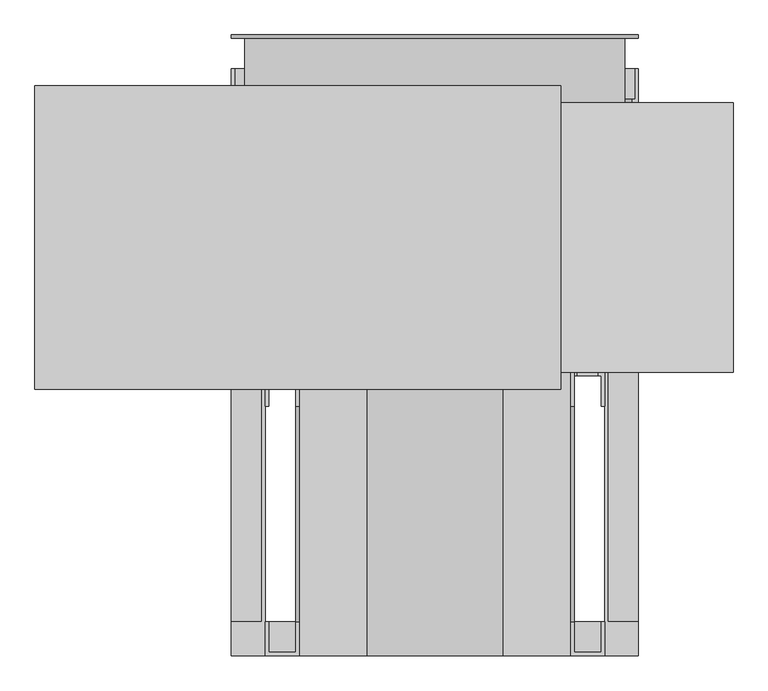
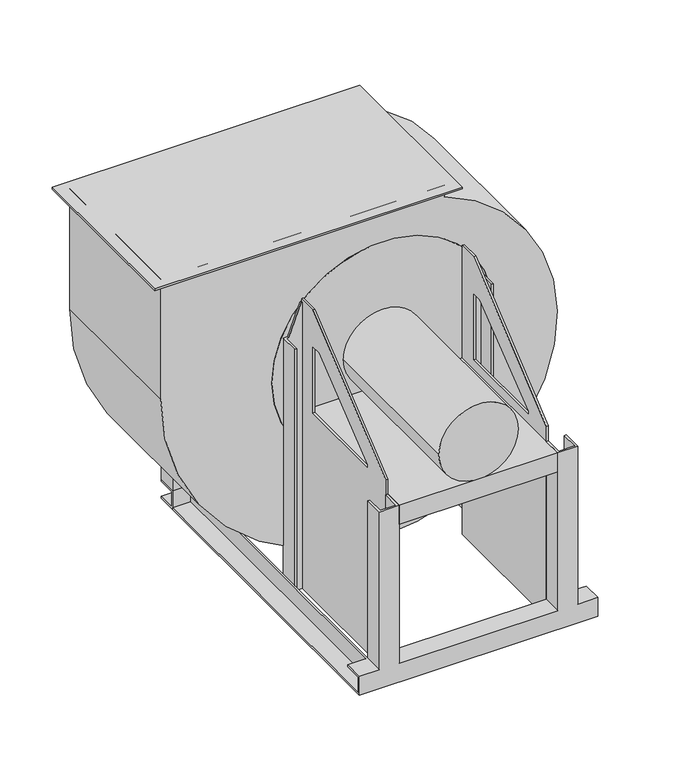
"""IFC4 building model written with IfcOpenShell, lengths in millimetres: proxy geometry, ВЕЗА_Вентилятор ВРАН : ВРАН6-056."""

from ifc_helpers import new_model, si_unit, point, frame, frame_2d, origin, place, context, project, spatial, polyline, circle_curve, trimmed, segment, composite_curve, outline, extrude, faceted_brep, source, transform, mapped, element, save


def mechanical_equipment_cec6a2f8(model_context):
    return source(origin(), model_context, "Body", "SolidModel", [
        extrude(outline(polyline([(185.5, -223.5), (-589.5, -223.5), (-589.5, 223.5), (185.5, 223.5), (185.5, -223.5)])), frame((0.0, 0.0, 940.0), z_axis=(0.0, 0.0, 1.0), x_axis=(1.0, 0.0, 0.0)), (0.0, 0.0, 1.0), 5.0),
        extrude(outline(composite_curve([segment(trimmed(circle_curve(frame_2d((625.0, 0.5002234)), 560.0002234), [point((625.0, -559.5))], [point((65.0, 0.0))], False, "CARTESIAN"), True, "CONTINUOUS"), segment(trimmed(circle_curve(frame_2d((504.1653304, 0.3189338)), 439.1654462), [point((65.0, 0.0))], [point((915.0, 155.5))], False, "CARTESIAN"), True, "CONTINUOUS"), segment(polyline([(915.0, 155.5), (945.0, 155.5), (945.0, -559.5), (625.0, -559.5)]), True, "CONTINUOUS")], self_intersect=False), holes=[composite_curve([segment(trimmed(circle_curve(frame_2d((570.0, 0.0)), 280.0), [point((570.0, -280.0))], [point((570.0, 280.0))], True, "CARTESIAN"), True, "CONTINUOUS"), segment(trimmed(circle_curve(frame_2d((570.0, 0.0)), 280.0), [point((570.0, 280.0))], [point((570.0, -280.0))], True, "CARTESIAN"), True, "CONTINUOUS")], self_intersect=False)]), frame((0.0, -198.5, 0.0), z_axis=(0.0, 1.0, 0.0), x_axis=(0.0, 0.0, 1.0)), (0.0, 0.0, 1.0), 397.0),
        faceted_brep([(-300.0, -611.5, 5.0), (-300.0, 198.5, 5.0), (-300.0, 198.5, 0.0), (-300.0, -616.5, 0.0), (-300.0, -616.5, 50.0), (-300.0, -566.5, 50.0), (-300.0, -566.5, 45.0), (-300.0, -611.5, 45.0), (300.0, -616.5, 50.0), (300.0, -616.5, 0.0), (300.0, 198.5, 0.0), (300.0, 198.5, 5.0), (300.0, -611.5, 5.0), (300.0, -611.5, 45.0), (300.0, -566.5, 45.0), (300.0, -566.5, 50.0), (-250.0, 198.5, 0.0), (-250.0, -566.5, 0.0), (250.0, -566.5, 0.0), (250.0, 198.5, 0.0), (-255.0, -566.5, 50.0), (-255.0, -566.5, 45.0), (255.0, -566.5, 45.0), (255.0, -566.5, 50.0), (-200.0, -566.5, 470.0), (-200.0, -566.5, 50.0), (200.0, -566.5, 50.0), (200.0, -566.5, 470.0), (205.0, -566.5, 470.0), (205.0, -566.5, 50.0), (245.0, -566.5, 50.0), (245.0, -566.5, 470.0), (250.0, -566.5, 470.0), (250.0, -566.5, 50.0), (-250.0, -566.5, 50.0), (-250.0, -566.5, 470.0), (-245.0, -566.5, 470.0), (-245.0, -566.5, 50.0), (-205.0, -566.5, 50.0), (-205.0, -566.5, 470.0), (205.0, -566.5, 5.0), (245.0, -566.5, 5.0), (245.0, -566.5, 45.0), (205.0, -566.5, 45.0), (-245.0, -566.5, 5.0), (-205.0, -566.5, 5.0), (-205.0, -566.5, 45.0), (-245.0, -566.5, 45.0), (-200.0, -566.5, 5.0), (200.0, -566.5, 5.0), (200.0, -566.5, 45.0), (-200.0, -566.5, 45.0), (-255.0, -611.5, 5.0), (-255.0, 198.5, 5.0), (255.0, 198.5, 5.0), (255.0, -611.5, 5.0), (205.0, -611.5, 5.0), (245.0, -611.5, 5.0), (-245.0, -611.5, 5.0), (-205.0, -611.5, 5.0), (-200.0, -611.5, 5.0), (200.0, -611.5, 5.0), (255.0, -611.5, 45.0), (-255.0, -611.5, 45.0), (205.0, -611.5, 45.0), (245.0, -611.5, 45.0), (-245.0, -611.5, 45.0), (-205.0, -611.5, 45.0), (-200.0, -611.5, 45.0), (200.0, -611.5, 45.0), (255.0, 198.5, 50.0), (250.0, 198.5, 50.0), (250.0, -616.5, 50.0), (-250.0, -616.5, 50.0), (-250.0, 198.5, 50.0), (-255.0, 198.5, 50.0), (205.0, -611.5, 50.0), (245.0, -611.5, 50.0), (-245.0, -611.5, 50.0), (-205.0, -611.5, 50.0), (-200.0, -616.5, 50.0), (200.0, -616.5, 50.0), (250.0, -616.5, 470.0), (200.0, -616.5, 470.0), (-200.0, -616.5, 470.0), (-250.0, -616.5, 470.0), (245.0, -611.5, 470.0), (205.0, -611.5, 470.0), (-205.0, -611.5, 470.0), (-245.0, -611.5, 470.0)], [[[0, 1, 2, 3, 4, 5, 6, 7]], [[8, 9, 10, 11, 12, 13, 14, 15]], [[10, 9, 3, 2, 16, 17, 18, 19]], [[5, 20, 21, 6]], [[14, 22, 23, 15]], [[24, 25, 26, 27, 28, 29, 30, 31, 32, 33, 18, 17, 34, 35, 36, 37, 38, 39], [40, 41, 42, 43], [44, 45, 46, 47], [48, 49, 50, 51]], [[1, 0, 52, 53]], [[54, 55, 12, 11]], [[40, 56, 57, 41]], [[44, 58, 59, 45]], [[48, 60, 61, 49]], [[12, 55, 62, 13]], [[7, 63, 52, 0]], [[56, 64, 65, 57]], [[58, 66, 67, 59]], [[60, 68, 69, 61]], [[6, 21, 63, 7]], [[13, 62, 22, 14]], [[64, 43, 42, 65]], [[66, 47, 46, 67]], [[68, 51, 50, 69]], [[15, 23, 70, 71, 33, 72, 8]], [[4, 73, 34, 74, 75, 20, 5]], [[29, 76, 77, 30]], [[37, 78, 79, 38]], [[25, 80, 81, 26]], [[8, 72, 82, 83, 81, 80, 84, 85, 73, 4, 3, 9]], [[70, 54, 11, 10, 19, 71]], [[70, 23, 22, 62, 55, 54]], [[19, 18, 33, 71]], [[75, 74, 16, 2, 1, 53]], [[53, 52, 63, 21, 20, 75]], [[74, 34, 17, 16]], [[83, 82, 32, 31, 86, 87, 28, 27]], [[84, 24, 39, 88, 89, 36, 35, 85]], [[86, 77, 76, 87]], [[31, 30, 77, 86]], [[41, 57, 65, 42]], [[82, 72, 33, 32]], [[27, 26, 81, 83]], [[49, 61, 69, 50]], [[43, 64, 56, 40]], [[87, 76, 29, 28]], [[35, 34, 73, 85]], [[47, 66, 58, 44]], [[89, 78, 37, 36]], [[88, 79, 78, 89]], [[39, 38, 79, 88]], [[45, 59, 67, 46]], [[51, 68, 60, 48]], [[84, 80, 25, 24]]]),
        extrude(outline(polyline([(-566.5, 0.0), (-566.5, 510.0420316), (-248.5420316, 770.0), (-198.5, 770.0), (-198.5, 0.0), (-566.5, 0.0)]), holes=[polyline([(-248.5, 495.0), (-248.5, 670.0), (-273.4504813, 670.0), (-486.5, 501.5949723), (-486.5, 495.0), (-248.5, 495.0)])]), frame((-205.0, 0.0, 0.0), z_axis=(1.0, 0.0, 0.0), x_axis=(0.0, 1.0, 0.0)), (0.0, 0.0, 1.0), 5.0),
        faceted_brep([(250.0, 198.5, 50.0), (250.0, 203.5, 50.0), (295.0, 203.5, 50.0), (295.0, 248.5, 50.0), (300.0, 248.5, 50.0), (300.0, 198.5, 50.0), (300.0, 198.5, 465.0), (289.966699, 198.5, 465.0), (258.2904546, 198.5, 370.0), (250.0, 198.5, 370.0), (300.0, 248.5, 465.0), (295.0, 248.5, 465.0), (295.0, 203.5, 465.0), (250.0, 203.5, 370.0), (258.2904546, 203.5, 370.0), (289.966699, 203.5, 465.0)], [[[0, 1, 2, 3, 4, 5]], [[5, 6, 7, 8, 9, 0]], [[4, 10, 6, 5]], [[3, 11, 10, 4]], [[2, 12, 11, 3]], [[1, 13, 14, 15, 12, 2]], [[0, 9, 13, 1]], [[14, 13, 9, 8]], [[8, 7, 15, 14]], [[7, 6, 10, 11, 12, 15]]]),
        faceted_brep([(-250.0, 198.5, 50.0), (-300.0, 198.5, 50.0), (-300.0, 248.5, 50.0), (-295.0, 248.5, 50.0), (-295.0, 203.5, 50.0), (-250.0, 203.5, 50.0), (-250.0, 203.5, 370.0), (-250.0, 198.5, 370.0), (-295.0, 203.5, 465.0), (-289.966699, 203.5, 465.0), (-258.2904546, 203.5, 370.0), (-295.0, 248.5, 465.0), (-300.0, 248.5, 465.0), (-300.0, 198.5, 465.0), (-258.2904546, 198.5, 370.0), (-289.966699, 198.5, 465.0)], [[[0, 1, 2, 3, 4, 5]], [[5, 6, 7, 0]], [[4, 8, 9, 10, 6, 5]], [[3, 11, 8, 4]], [[2, 12, 11, 3]], [[1, 13, 12, 2]], [[0, 7, 14, 15, 13, 1]], [[9, 8, 11, 12, 13, 15]], [[15, 14, 10, 9]], [[14, 7, 6, 10]]]),
        extrude(outline(polyline([(-566.5, 0.0), (-566.5, 510.0420316), (-248.5420316, 770.0), (-198.5, 770.0), (-198.5, 0.0), (-566.5, 0.0)]), holes=[polyline([(-248.5, 495.0), (-248.5, 670.0), (-273.4504813, 670.0), (-486.5, 501.5949723), (-486.5, 495.0), (-248.5, 495.0)])]), frame((200.0, 0.0, 0.0), z_axis=(1.0, 0.0, 0.0), x_axis=(0.0, 1.0, 0.0)), (0.0, 0.0, 1.0), 5.0),
        faceted_brep([(200.0, -198.5, 0.0), (250.0, -198.5, 0.0), (250.0, -248.5, 0.0), (245.0, -248.5, 0.0), (245.0, -203.5, 0.0), (200.0, -203.5, 0.0), (200.0, -198.5, 763.6095143), (208.75409, -198.5, 763.6095143), (240.0, -198.5, 680.0), (250.0, -198.5, 680.0), (250.0, -248.5, 680.0), (245.0, -248.5, 680.0), (245.0, -203.5, 680.0), (240.0, -203.5, 680.0), (208.75409, -203.5, 763.6095143), (200.0, -203.5, 763.6095143)], [[[0, 1, 2, 3, 4, 5]], [[0, 6, 7, 8, 9, 1]], [[1, 9, 10, 2]], [[2, 10, 11, 3]], [[3, 11, 12, 4]], [[4, 12, 13, 14, 15, 5]], [[5, 15, 6, 0]], [[7, 6, 15, 14]], [[14, 13, 8, 7]], [[13, 12, 11, 10, 9, 8]]]),
        faceted_brep([(-200.0, -198.5, 0.0), (-200.0, -203.5, 0.0), (-245.0, -203.5, 0.0), (-245.0, -248.5, 0.0), (-250.0, -248.5, 0.0), (-250.0, -198.5, 0.0), (-200.0, -198.5, 763.6095143), (-200.0, -203.5, 763.6095143), (-208.75409, -203.5, 763.6095143), (-240.0, -203.5, 680.0), (-245.0, -203.5, 680.0), (-245.0, -248.5, 680.0), (-250.0, -248.5, 680.0), (-250.0, -198.5, 680.0), (-240.0, -198.5, 680.0), (-208.75409, -198.5, 763.6095143)], [[[0, 1, 2, 3, 4, 5]], [[0, 6, 7, 1]], [[1, 7, 8, 9, 10, 2]], [[2, 10, 11, 3]], [[3, 11, 12, 4]], [[4, 12, 13, 5]], [[5, 13, 14, 15, 6, 0]], [[14, 13, 12, 11, 10, 9]], [[9, 8, 15, 14]], [[8, 7, 6, 15]]]),
        extrude(outline(polyline([(198.5, 50.0), (248.5, 50.0), (248.5, 45.0), (203.5, 45.0), (203.5, 5.0), (248.5, 5.0), (248.5, 0.0), (198.5, 0.0), (198.5, 50.0)])), frame((-300.0, 0.0, 0.0), z_axis=(1.0, 0.0, 0.0), x_axis=(0.0, 1.0, 0.0)), (0.0, 0.0, 1.0), 600.0),
        extrude(outline(composite_curve([segment(trimmed(circle_curve(frame_2d((570.0, 0.0)), 280.0), [point((570.0, -280.0))], [point((570.0, 280.0))], False, "CARTESIAN"), True, "CONTINUOUS"), segment(trimmed(circle_curve(frame_2d((570.0, 0.0)), 280.0), [point((570.0, 280.0))], [point((570.0, -280.0))], False, "CARTESIAN"), True, "CONTINUOUS")], self_intersect=False)), frame((0.0, -198.5, 0.0), z_axis=(0.0, 1.0, 0.0), x_axis=(0.0, 0.0, 1.0)), (0.0, 0.0, 1.0), 5.0),
        extrude(outline(composite_curve([segment(trimmed(circle_curve(frame_2d((570.0, 0.0)), 300.0), [point((570.0, -300.0))], [point((570.0, 300.0))], False, "CARTESIAN"), True, "CONTINUOUS"), segment(trimmed(circle_curve(frame_2d((570.0, 0.0)), 300.0), [point((570.0, 300.0))], [point((570.0, -300.0))], False, "CARTESIAN"), True, "CONTINUOUS")], self_intersect=False), holes=[composite_curve([segment(trimmed(circle_curve(frame_2d((570.0, 0.0)), 270.0), [point((570.0, -270.0))], [point((570.0, 270.0))], True, "CARTESIAN"), True, "CONTINUOUS"), segment(trimmed(circle_curve(frame_2d((570.0, 0.0)), 270.0), [point((570.0, 270.0))], [point((570.0, -270.0))], True, "CARTESIAN"), True, "CONTINUOUS")], self_intersect=False)]), frame((0.0, 293.5, 0.0), z_axis=(0.0, 1.0, 0.0), x_axis=(0.0, 0.0, 1.0)), (0.0, 0.0, 1.0), 5.0),
        extrude(outline(polyline([(200.0, -616.5), (-200.0, -616.5), (-200.0, -198.5), (200.0, -198.5), (200.0, -616.5)])), frame((0.0, 0.0, 420.0), z_axis=(0.0, 0.0, 1.0), x_axis=(1.0, 0.0, 0.0)), (0.0, 0.0, 1.0), 50.0),
        extrude(outline(composite_curve([segment(trimmed(circle_curve(frame_2d((570.0, 0.0)), 100.0), [point((570.0, 100.0))], [point((570.0, -100.0))], False, "CARTESIAN"), True, "CONTINUOUS"), segment(trimmed(circle_curve(frame_2d((570.0, 0.0)), 100.0), [point((570.0, -100.0))], [point((570.0, 100.0))], False, "CARTESIAN"), True, "CONTINUOUS")], self_intersect=False)), frame((0.0, -616.5, 0.0), z_axis=(0.0, 1.0, 0.0), x_axis=(0.0, 0.0, 1.0)), (0.0, 0.0, 1.0), 418.0),
        extrude(outline(composite_curve([segment(trimmed(circle_curve(frame_2d((570.0, 0.0)), 280.0), [point((570.0, 280.0))], [point((570.0, -280.0))], False, "CARTESIAN"), True, "CONTINUOUS"), segment(trimmed(circle_curve(frame_2d((570.0, 0.0)), 280.0), [point((570.0, -280.0))], [point((570.0, 280.0))], False, "CARTESIAN"), True, "CONTINUOUS")], self_intersect=False), holes=[composite_curve([segment(trimmed(circle_curve(frame_2d((570.0, 0.0)), 270.0), [point((570.0, 270.0))], [point((570.0, -270.0))], True, "CARTESIAN"), True, "CONTINUOUS"), segment(trimmed(circle_curve(frame_2d((570.0, 0.0)), 270.0), [point((570.0, -270.0))], [point((570.0, 270.0))], True, "CARTESIAN"), True, "CONTINUOUS")], self_intersect=False)]), frame((0.0, 198.5, 0.0), z_axis=(0.0, 1.0, 0.0), x_axis=(0.0, 0.0, 1.0)), (0.0, 0.0, 1.0), 100.0),
    ])


if __name__ == "__main__":
    model = new_model("IFC4")
    model_context = context("Model", 3, world=origin())
    ifc_project = project(units=[si_unit("LENGTHUNIT", "METRE", prefix="MILLI")], contexts=[model_context])
    site = spatial("IfcSite", under=ifc_project)
    building = spatial("IfcBuilding", under=site)
    placement = place(None, origin())
    mechanical_equipment_shape = mechanical_equipment_cec6a2f8(model_context)
    element("IfcBuildingElementProxy", 1, Name="ВЕЗА_Вентилятор ВРАН : ВРАН6-056", ObjectType="ВЕЗА_Вентилятор ВРАН : ВРАН6-056", at=placement, inside=building, context=model_context, shape_type="MappedRepresentation", body=[
        mapped(mechanical_equipment_shape, transform((0.0, 0.0, 0.0), x_axis=(1.0, 0.0, 0.0), y_axis=(0.0, 1.0, 0.0), z_axis=(0.0, 0.0, 1.0))),
    ])
    save(model, "model.ifc")

# Revit data of these elements
# Type "ВЕЗА_Вентилятор ВРАН : ВРАН6-056"
#   УголВысота = "ВРАН_Угол_Высота"
#   ADSK_Этаж [instance default] = ""
#   ADSK_Примечание [instance default] = ""
#   ADSK_Позиция = "9"
#   ADSK_Обозначение = ""
#   ADSK_Наименование = "Вентилятор радиальный ВРАН6; типоразмер 056; режим работы Т80; исполнение взрывозащищенное коррозионностойкое; номинальная мощность Nном=2,2кВт, число полюсов 4; климатическое исполнение УХЛ2; конструктивное исполнение 1; положение корпуса ПО; без ТШК"
#   О_Назначение [instance default] = ""
#   ADSK_Марка = "ВРАН6-056-Т80-ВК1-00220/4-УХЛ2-1-ПО-О ТУ 4861-104-40149153-2007"
#   ADSK_Комплект [instance default] = ""
#   ADSK_Код изделия = "4039929"
#   ADSK_Зона [instance default] = ""
#   ADSK_Единица измерения = "компл."
#   И_НаименованиеФитинга = ""
#   И_НаименованиеСистемы [instance default] = ""
#   И_КодОборудования = "ВРАН6-056-П0-0"
#   ADSK_Завод-изготовитель = "ООО \"Веза\", Россия, Москва, ИНН 505001001, info@veza.ru"
#   Габариты = "vran_du"
#   ШиринаСтойкиОкна2 = 100 mm
#   ШиринаСтойкиОкна1 = 130 mm
#   ШиринаСтойкиДвигателя = 50 mm
#   Уголок = 50 mm
#   УголНаклона [instance default] = 0°
#   Угол [instance default] = 0°
#   Столик = -50 mm
#   Расход [instance default] = 0 m³/h
#   ADSK_Масса = 100
#   ADSK_Количество = 1
#   ADSK_Номинальная мощность [instance default] = 0 W
#   РадиусДвигателя = 100 mm
#   НомерВентилятора = 5.6 mm
#   ВысотаПлощадкиДвигателя [instance default] = 470 mm
#   ВерхОпор = 200 mm
#   R3 = 300 mm
#   R2 = 270 mm
#   Lmax = 865 mm
#   h [instance default] = 570 mm
#   R = 280 mm
#   L2 = 202 mm
#   H = 945 mm
#   D = 560 mm
#   C = 550 mm
#   B_корпуса = 1020 mm
#   B = 720 mm
#   A = 397 mm
#   Швеллер = yes
#   Default Elevation = 0
#   Type Comments = ""
